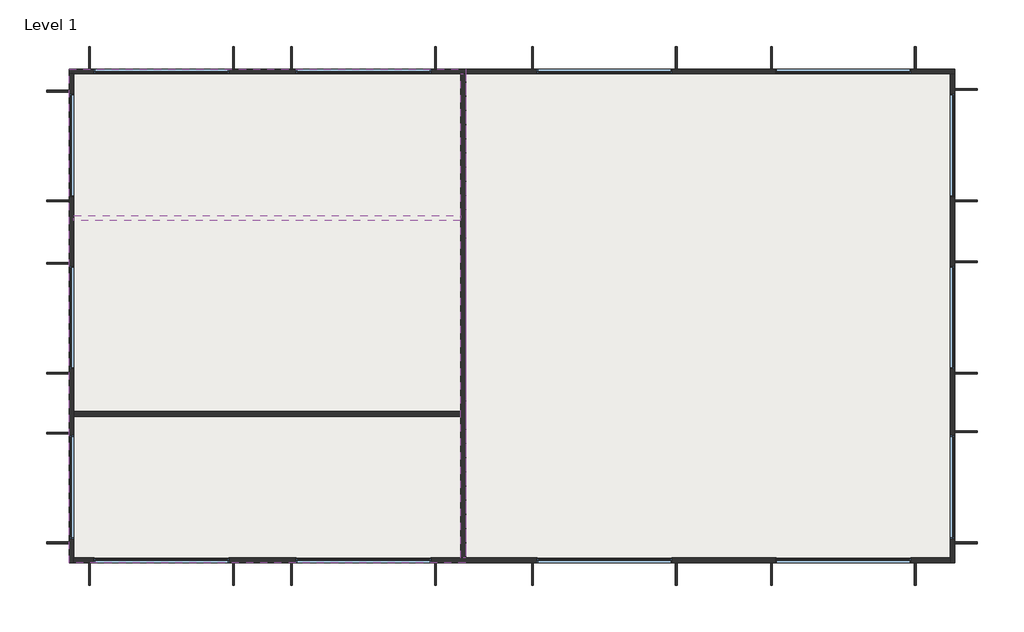
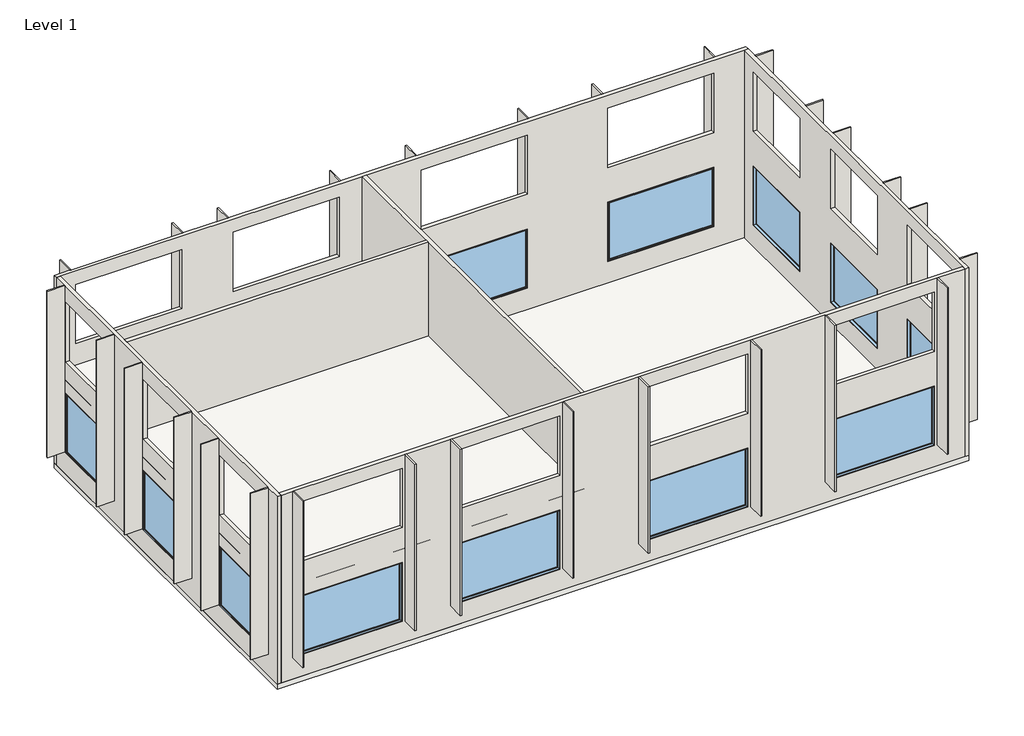
# One storey: 36 walls, 14 windows, 2 slabs.
# Revit data of these elements (continued)
# Type "M_Fixed : 2500x 3220mm" (continued)
#   Default Sill Height = 305 mm
#   Width = 3219.6 mm
#   Window Inset = 19 mm
#   Frame Exterior Material = Sash
#   Frame Interior Material = Sash
#   Glass Pane Material = Glass
#   Sash = Sash
#   Wall Closure = (empty or 0)
# Element 1 (IfcSlab, "160mm Concrete With 50mm Metal Deck")
#   Height Offset From Level = 0 mm
#   Phase Created = New Construction
#   Materials on its faces: "Metal Deck", "Default Floor"
# Element 2 (IfcSlab, "160mm Concrete With 50mm Metal Deck")
#   Height Offset From Level = 3962.4 mm
#   Phase Created = New Construction
#   Materials on its faces: "Metal Deck", "Default Floor"
# Elements 3, 4, 5, 6 (IfcWall, "Generic - 152.4mm")
#   Top Offset = 0 mm
#   Base Offset = 0 mm
#   wall height = 7924.8 mm
#   Phase Created = New Construction
#   Base Constraint = Level 1
#   Top Constraint = Roof Level
#   Materials on its faces: "Default Wall"
# Element 7 (IfcWall, "Generic - 152.4mm - Interior")
#   Top Offset = 3962.4 mm
#   Base Offset = 0 mm
#   wall height = 3752.4 mm
#   Phase Created = New Construction
#   Base Constraint = Level 1
#   Top Constraint = Level 1
#   Materials on its faces: "Default Wall"
# Element 8 (IfcWall, "Generic - 152.4mm - Interior")
#   Top Offset = 3862.4 mm
#   Base Offset = 0 mm
#   wall height = 3752.4 mm
#   Phase Created = New Construction
#   Base Constraint = Level 1
#   Top Constraint = Level 1
#   Materials on its faces: "Default Wall"
# Elements 9, 10 (IfcWall, "Generic - 152.4mm - Interior")
#   built-in parameter 1001111 = 3962.4 mm
#   Top Offset = 0 mm
#   Base Offset = 3962.4 mm
#   Unconnected Height = 3962.4 mm
#   wall height = 3962.4 mm
#   Phase Created = New Construction
#   Base Constraint = Level 1
#   Top Constraint = Roof Level
#   Materials on its faces: "Default Wall"
# Elements 11, 12, 13, 14, 15, 16, 17, 18, 19, 20, 21, 22, 23, 24, 25, 26, 27, 28, 29, 30, 31, 32, 33, 34, 35, 36, 37, 38 (IfcWall, "Shading devices")
#   built-in parameter 1001111 = 902.4 mm
#   Top Offset = 0 mm
#   Base Offset = 902.4 mm
#   wall height = 7022.4 mm
#   Phase Created = New Construction
#   Base Constraint = Level 1
#   Top Constraint = Roof Level
#   Materials on its faces: "Default Wall"
# Element 39 (IfcWindow, "M_Fixed : 2500X 4228mm")
#   Mark = "10"
#   Phase Created = New Construction
#   Materials on its faces: "Sash", "Glass"
# Element 40 (IfcWindow, "M_Fixed : 2500X 4228mm")
#   Mark = "11"
#   Phase Created = New Construction
#   Materials on its faces: "Sash", "Glass"
# Element 41 (IfcWindow, "M_Fixed : 2500X 4228mm")
#   Mark = "12"
#   Phase Created = New Construction
#   Materials on its faces: "Sash", "Glass"
# Element 42 (IfcWindow, "M_Fixed : 2500X 4228mm")
#   Mark = "13"
#   Phase Created = New Construction
#   Materials on its faces: "Sash", "Glass"
# Element 43 (IfcWindow, "M_Fixed : 2500X 4228mm")
#   Mark = "14"
#   Phase Created = New Construction
#   Materials on its faces: "Sash", "Glass"
# Element 44 (IfcWindow, "M_Fixed : 2500X 4228mm")
#   Mark = "15"
#   Phase Created = New Construction
#   Materials on its faces: "Sash", "Glass"
# Element 45 (IfcWindow, "M_Fixed : 2500X 4228mm")
#   Mark = "16"
#   Phase Created = New Construction
#   Materials on its faces: "Sash", "Glass"
# Element 46 (IfcWindow, "M_Fixed : 2500X 4228mm")
#   Mark = "17"
#   Phase Created = New Construction
#   Materials on its faces: "Sash", "Glass"
# Element 47 (IfcWindow, "M_Fixed : 2500x 3220mm")
#   Mark = "26"
#   Phase Created = New Construction
#   Materials on its faces: "Sash", "Glass"
# Element 48 (IfcWindow, "M_Fixed : 2500x 3220mm")
#   Mark = "28"
#   Phase Created = New Construction
#   Materials on its faces: "Sash", "Glass"
# Element 49 (IfcWindow, "M_Fixed : 2500x 3220mm")
#   Mark = "29"
#   Phase Created = New Construction
#   Materials on its faces: "Sash", "Glass"
# Element 50 (IfcWindow, "M_Fixed : 2500x 3220mm")
#   Mark = "30"
#   Phase Created = New Construction
#   Materials on its faces: "Sash", "Glass"
# Element 51 (IfcWindow, "M_Fixed : 2500x 3220mm")
#   Mark = "31"
#   Phase Created = New Construction
#   Materials on its faces: "Sash", "Glass"
# Element 52 (IfcWindow, "M_Fixed : 2500x 3220mm")
#   Mark = "32"
#   Phase Created = New Construction
#   Materials on its faces: "Sash", "Glass"
# Materials
#   "Metal Deck": class "Metal", colour RGB 247 247 247, transparency 0, Description = "Steel, mill finish", Cost = 0
#   "Sash": class "Wood", colour RGB 136 99 55, transparency 0
#   "Glass": class "Glass", colour RGB 0 128 192, transparency 0.9, Description = "Soda Lime Glass", Cost = 0
#   "Default Floor": class "Miscellaneous", colour RGB 127 127 127, transparency 0, Cost = 0
#   "Default Wall": class "Miscellaneous", colour RGB 128 128 128, transparency 0, Cost = 0
# Room at (7259.725, -1600.456) mm, phase "New Construction", upper level "Level 2", upper offset 0 mm, lower offset 0 mm
#   Number = "6"
#   Name = "Room"
# Room at (8198.725, 4816.984) mm, phase "New Construction", upper level "Level 2", upper offset 0 mm, lower offset 0 mm
#   Number = "7"
#   Name = "Room"
# Room at (21274.823, 2677.837) mm, phase "New Construction", upper level "Roof Level", upper offset 0 mm, lower offset 0 mm
#   Number = "8"
#   Name = "Room"
